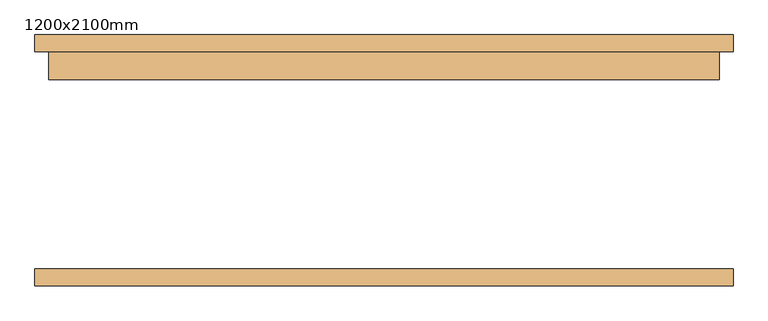
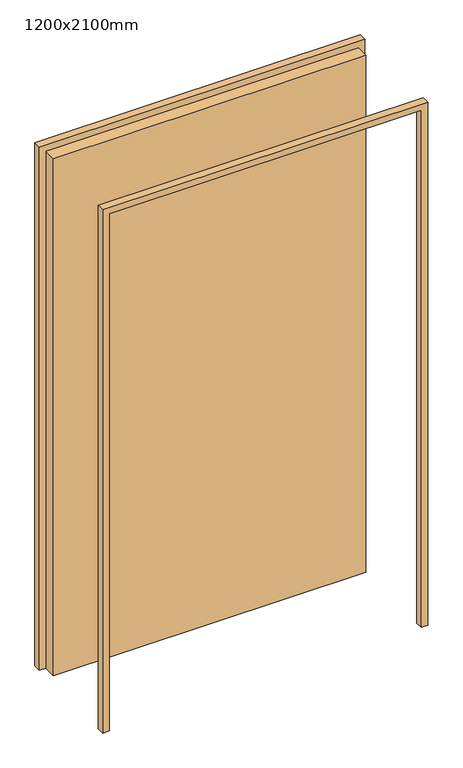
"""IFC4 building model written with IfcOpenShell, lengths in millimetres: door geometry, WWm-SingleSolid-Flush : 1200x2100mm."""

from ifc_helpers import new_model, si_unit, frame, origin, origin_with_axes, place, context, project, spatial, polyline, outline, extrude, source, transform, mapped, element, save


def door_1200x2100mm_edb93628(model_context):
    return source(origin(), model_context, "Body", "SweptSolid", [
        extrude(outline(polyline([(2125.0, -625.0), (0.0, -625.0), (0.0, -600.0), (2100.0, -600.0), (2100.0, 600.0), (0.0, 600.0), (0.0, 625.0), (2125.0, 625.0), (2125.0, -625.0)])), frame((0.0, 195.0, 0.0), z_axis=(0.0, 1.0, 0.0), x_axis=(0.0, 0.0, 1.0)), (0.0, 0.0, 1.0), 30.0),
        extrude(outline(polyline([(2125.0, 625.0), (2125.0, -625.0), (0.0, -625.0), (0.0, -600.0), (2100.0, -600.0), (2100.0, 600.0), (0.0, 600.0), (0.0, 625.0), (2125.0, 625.0)])), frame((0.0, -225.0, 0.0), z_axis=(0.0, 1.0, 0.0), x_axis=(0.0, 0.0, 1.0)), (0.0, 0.0, 1.0), 30.0),
        extrude(outline(polyline([(600.0, 145.0), (-600.0, 145.0), (-600.0, 195.0), (600.0, 195.0), (600.0, 145.0)])), origin_with_axes(), (0.0, 0.0, 1.0), 2100.0),
    ])


if __name__ == "__main__":
    model = new_model("IFC4")
    model_context = context("Model", 3, world=origin())
    ifc_project = project(units=[si_unit("LENGTHUNIT", "METRE", prefix="MILLI")], contexts=[model_context])
    site = spatial("IfcSite", under=ifc_project)
    building = spatial("IfcBuilding", under=site)
    placement = place(None, origin())
    door_1200x2100mm_shape = door_1200x2100mm_edb93628(model_context)
    element("IfcDoor", 1, ObjectType="WWm-SingleSolid-Flush : 1200x2100mm", at=placement, inside=building, context=model_context, shape_type="MappedRepresentation", body=[
        mapped(door_1200x2100mm_shape, transform((0.0, 0.0, 0.0), x_axis=(1.0, 0.0, 0.0), y_axis=(0.0, 1.0, 0.0), z_axis=(0.0, 0.0, 1.0))),
    ])
    save(model, "model.ifc")

# Revit data of these elements
# Type "WWm-SingleSolid-Flush : 1200x2100mm"
#   Type Mark = "EX1-55"
#   Construction Type Id = "MDOOR"
#   Assembly Code = "C1020"
#   Analytic Construction = "Metal"
#   Thickness = 50 mm
#   Thermal Resistance (R) = 0.270117 (m²·K)/W
#   Heat Transfer Coefficient (U) = 3.7021 W/(m²·K)
#   Height = 2100 mm
#   Trim Projection Ext = 30 mm
#   Trim Projection Int = 30 mm
#   Trim Width = 25 mm
#   Width = 1200 mm
#   Not 90 Degree [instance default] = no
#   90 Degree [instance default] = yes
#   Door Material = WW-EC-RGB-White
#   Frame Material = WW-EC-RGB-White
#   Visual Light Transmittance = 0
#   Solar Heat Gain Coefficient = 0
#   Function = (empty or 0)
#   Wall Closure = (empty or 0)
# Element 1 (IfcDoor, "WWm-SingleSolid-Flush : 1200x2100mm")
#   Materials on its faces: "WW-EC-RGB-White"
# Materials
#   "WW-EC-RGB-White": class "Generic", colour RGB 255 255 255, transparency 0, Comments = "If region requests off-white, swith asset color to RGB 231-228-220", Description = "Generic Color", Cost = 0
